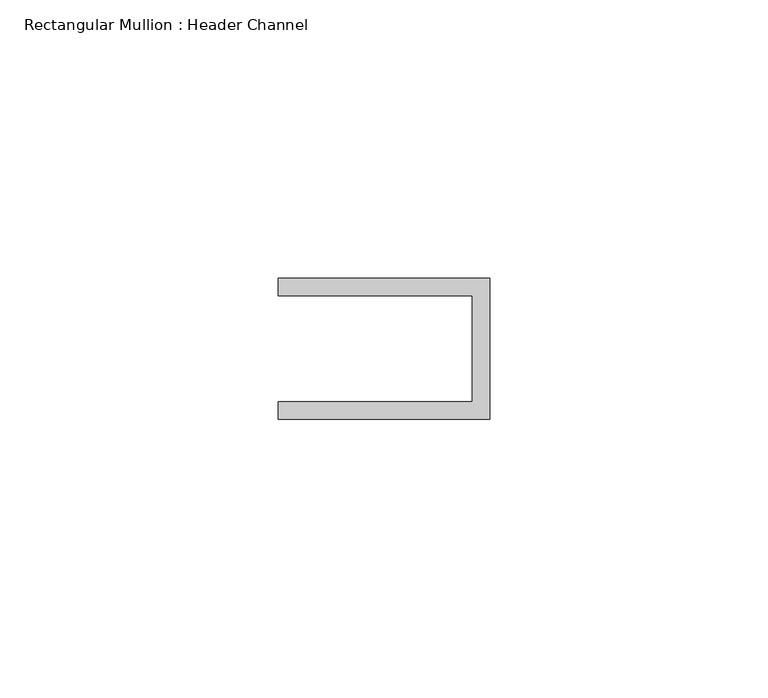
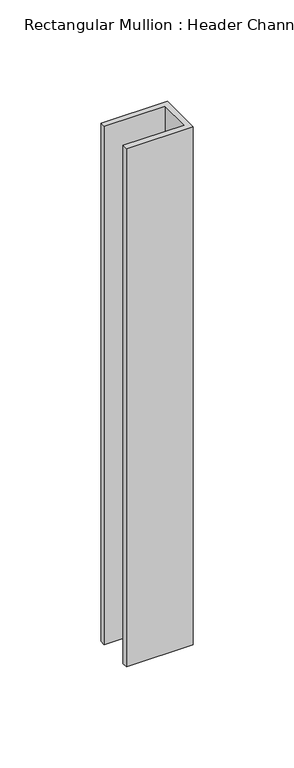
"""IFC4 building model written with IfcOpenShell, lengths in millimetres: member geometry, Rectangular Mullion : Header Channel."""

from ifc_helpers import new_model, si_unit, frame, origin, place, context, project, spatial, polyline, outline, extrude, source, transform, mapped, element, save


def rectangular_mullion_header_channel_30638dab(model_context):
    return source(origin(), model_context, "Body", "SweptSolid", [
        extrude(outline(polyline([(0.0, -12.7), (-38.1, -12.7), (-38.1, -9.525), (-3.175, -9.525), (-3.175, 9.525), (-38.1, 9.525), (-38.1, 12.7), (0.0, 12.7), (0.0, -12.7)])), frame((0.0, 0.0, -313.2666667), z_axis=(0.0, 0.0, 1.0), x_axis=(1.0, 0.0, 0.0)), (0.0, 0.0, 1.0), 313.2666667),
    ])


if __name__ == "__main__":
    model = new_model("IFC4")
    model_context = context("Model", 3, world=origin())
    ifc_project = project(units=[si_unit("LENGTHUNIT", "METRE", prefix="MILLI")], contexts=[model_context])
    site = spatial("IfcSite", under=ifc_project)
    building = spatial("IfcBuilding", under=site)
    placement = place(None, origin())
    rectangular_mullion_header_channel_shape = rectangular_mullion_header_channel_30638dab(model_context)
    element("IfcMember", 1, ObjectType="Rectangular Mullion : Header Channel", at=placement, inside=building, context=model_context, shape_type="MappedRepresentation", body=[
        mapped(rectangular_mullion_header_channel_shape, transform((0.0, 0.0, 0.0), x_axis=(1.0, 0.0, 0.0), y_axis=(0.0, 1.0, 0.0), z_axis=(0.0, 0.0, 1.0))),
    ])
    save(model, "model.ifc")

# Revit data of these elements
# Type "Rectangular Mullion : Header Channel"
#   built-in parameter 1007322 = 0.0833333 (stored number, unit not read)
#   built-in parameter 1007321 = -0.03125 (stored number, unit not read)
#   built-in parameter 1007320 = 0.0416667 (stored number, unit not read)
# Element 1 (IfcMember, "Rectangular Mullion : Header Channel")
#   Materials on its faces: "ALUM"
# Materials
#   "ALUM": class "Generic", colour RGB 157 157 157, transparency 0, Cost = 0
